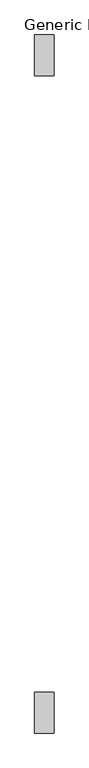
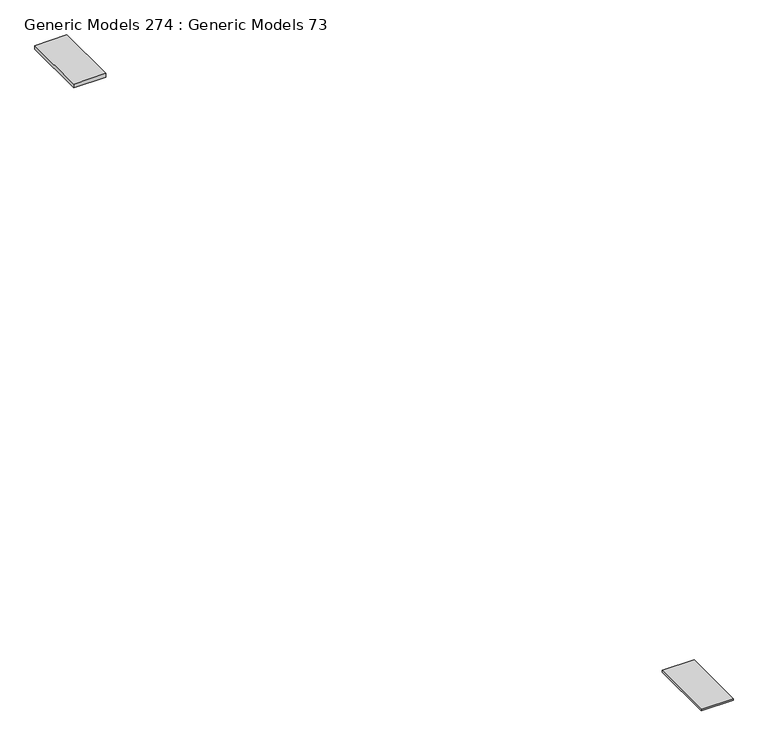
"""IFC4 building model written with IfcOpenShell, lengths in millimetres: proxy geometry, Generic Models 274 : Generic Models 73."""

from ifc_helpers import new_model, si_unit, frame, origin, place, context, project, spatial, polyline, outline, extrude, source, transform, mapped, element, save


def generic_models_274_generic_models_73_644cdb5e(model_context):
    return source(origin(), model_context, "Body", "SweptSolid", [
        extrude(outline(polyline([(32053.2090778, 30964.2606313), (32053.2090778, 30690.2031612), (31923.0340778, 30690.2031612), (31923.0340778, 30964.2606313), (32053.2090778, 30964.2606313)])), frame((0.0, 0.0, 266414.25), z_axis=(0.0, 0.0, 1.0), x_axis=(1.0, 0.0, 0.0)), (0.0, 0.0, 1.0), 7.9375),
        extrude(outline(polyline([(32053.2090778, 35373.9582942), (32053.2090778, 35100.8368035), (31923.0340778, 35100.8368035), (31923.0340778, 35373.9582942), (32053.2090778, 35373.9582942)])), frame((0.0, 0.0, 266414.25), z_axis=(0.0, 0.0, 1.0), x_axis=(1.0, 0.0, 0.0)), (0.0, 0.0, 1.0), 15.875),
    ])


if __name__ == "__main__":
    model = new_model("IFC4")
    model_context = context("Model", 3, world=origin())
    ifc_project = project(units=[si_unit("LENGTHUNIT", "METRE", prefix="MILLI")], contexts=[model_context])
    site = spatial("IfcSite", under=ifc_project)
    building = spatial("IfcBuilding", under=site)
    placement = place(None, origin())
    generic_models_274_generic_models_73_shape = generic_models_274_generic_models_73_644cdb5e(model_context)
    element("IfcBuildingElementProxy", 1, Name="Generic Models 274 : Generic Models 73", ObjectType="Generic Models 274 : Generic Models 73", at=placement, inside=building, context=model_context, shape_type="MappedRepresentation", body=[
        mapped(generic_models_274_generic_models_73_shape, transform((0.0, 0.0, 0.0), x_axis=(1.0, 0.0, 0.0), y_axis=(0.0, 1.0, 0.0), z_axis=(0.0, 0.0, 1.0))),
    ])
    save(model, "model.ifc")

# Revit data of these elements
# Element 1 (IfcBuildingElementProxy, "Generic Models 274 : Generic Models 73")
#   Materials on its faces: "6 x 5/8\" BASE PL. W/ (2) \n5/8\" EMBEDMENT EPOXY ANCHORS"
# Materials
#   "6 x 5/8\" BASE PL. W/ (2) \n5/8\" EMBEDMENT EPOXY ANCHORS": class "Metal", colour RGB 199 199 199, transparency 0, Description = "Carbon steel", Cost = 0
